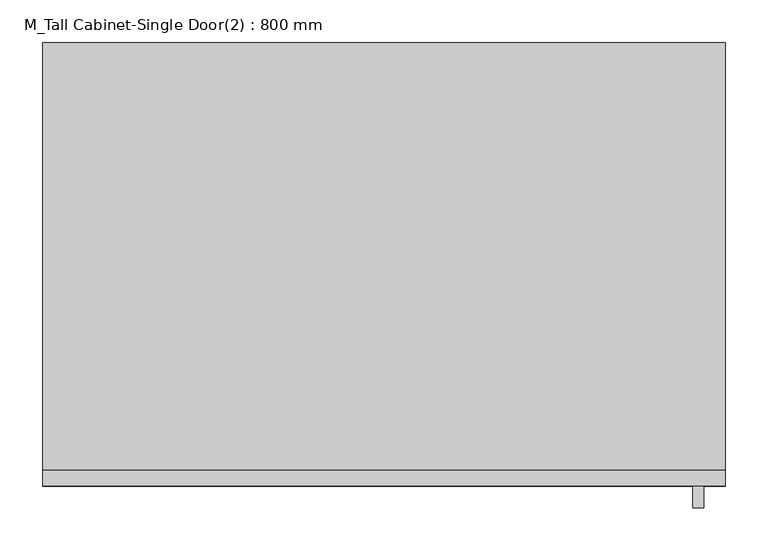
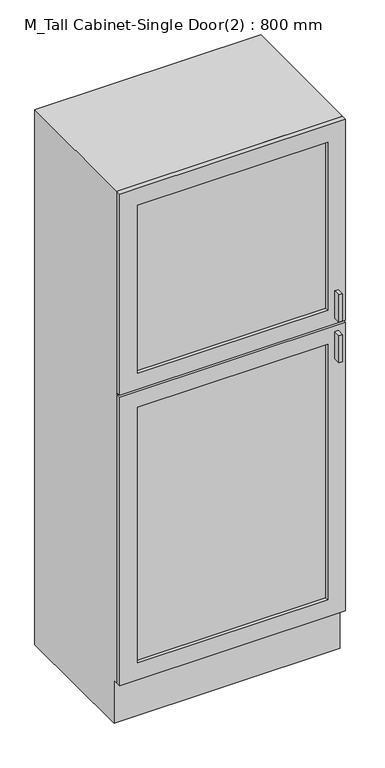
"""IFC4 building model written with IfcOpenShell, lengths in millimetres: furniture geometry, M_Tall Cabinet-Single Door(2) : 800 mm."""

from ifc_helpers import new_model, si_unit, frame, origin, place, context, project, spatial, polyline, outline, extrude, faceted_brep, source, transform, mapped, element, save


def m_tall_cabinet_single_door_2_800_mm_91498984(model_context):
    return source(origin(), model_context, "Body", "SolidModel", [
        faceted_brep([(418.7377049, -500.95, 161.5875), (418.7377049, -500.95, 2000.0), (-381.2622951, -500.95, 2000.0), (-381.2622951, -500.95, 161.5875), (399.6877049, -500.95, 1980.95), (399.6877049, -500.95, 180.6375), (-362.2122951, -500.95, 180.6375), (-362.2122951, -500.95, 1980.95), (-381.2622951, 0.0, 2000.0), (418.7377049, 0.0, 2000.0), (418.7377049, 0.0, 0.0), (-381.2622951, 0.0, 0.0), (399.6877049, 0.0, 1980.95), (-362.2122951, 0.0, 1980.95), (-362.2122951, 0.0, 180.6375), (399.6877049, 0.0, 180.6375), (418.7377049, -485.0, 161.5875), (418.7377049, -485.0, 0.0), (-381.2622951, -485.0, 0.0), (-381.2622951, -485.0, 161.5875)], [[[0, 1, 2, 3], [4, 5, 6, 7]], [[8, 9, 10, 11], [12, 13, 14, 15]], [[1, 0, 16, 17, 10, 9]], [[2, 1, 9, 8]], [[3, 2, 8, 11, 18, 19]], [[0, 3, 19, 16]], [[5, 4, 12, 15]], [[6, 5, 15, 14]], [[7, 6, 14, 13]], [[4, 7, 13, 12]], [[10, 17, 18, 11]], [[18, 17, 16, 19]]]),
        extrude(outline(polyline([(393.3377049, -545.4), (380.8054733, -545.4), (380.8054733, -520.0), (393.3377049, -520.0), (393.3377049, -545.4)])), frame((0.0, 0.0, 1269.9480367), z_axis=(0.0, 0.0, 1.0), x_axis=(1.0, 0.0, 0.0)), (0.0, 0.0, 1.0), 101.6),
        extrude(outline(polyline([(393.3377049, -545.4), (380.8054733, -545.4), (380.8054733, -520.0), (393.3377049, -520.0), (393.3377049, -545.4)])), frame((0.0, 0.0, 1117.5480367), z_axis=(0.0, 0.0, 1.0), x_axis=(1.0, 0.0, 0.0)), (0.0, 0.0, 1.0), 101.6),
        extrude(outline(polyline([(355.2377049, -507.3), (-317.7622951, -507.3), (-317.7622951, -500.95), (355.2377049, -500.95), (355.2377049, -507.3)])), frame((0.0, 0.0, 1308.0480367), z_axis=(0.0, 0.0, 1.0), x_axis=(1.0, 0.0, 0.0)), (0.0, 0.0, 1.0), 628.4519633),
        extrude(outline(polyline([(355.2377049, -507.3), (-317.7622951, -507.3), (-317.7622951, -500.95), (355.2377049, -500.95), (355.2377049, -507.3)])), frame((0.0, 0.0, 225.0875), z_axis=(0.0, 0.0, 1.0), x_axis=(1.0, 0.0, 0.0)), (0.0, 0.0, 1.0), 955.9605367),
        extrude(outline(polyline([(2000.0, 418.7377049), (2000.0, -381.2622951), (1247.7230367, -381.2622951), (1247.7230367, 418.7377049), (2000.0, 418.7377049)]), holes=[polyline([(1936.5, 355.2377049), (1308.0480367, 355.2377049), (1308.0480367, -317.7622951), (1936.5, -317.7622951), (1936.5, 355.2377049)])]), frame((0.0, -520.0, 0.0), z_axis=(0.0, 1.0, 0.0), x_axis=(0.0, 0.0, 1.0)), (0.0, 0.0, 1.0), 19.05),
        extrude(outline(polyline([(161.5875, 418.7377049), (1241.3730367, 418.7377049), (1241.3730367, -381.2622951), (161.5875, -381.2622951), (161.5875, 418.7377049)]), holes=[polyline([(1181.0480367, 355.2377049), (225.0875, 355.2377049), (225.0875, -317.7622951), (1181.0480367, -317.7622951), (1181.0480367, 355.2377049)])]), frame((0.0, -520.0, 0.0), z_axis=(0.0, 1.0, 0.0), x_axis=(0.0, 0.0, 1.0)), (0.0, 0.0, 1.0), 19.05),
        extrude(outline(polyline([(399.6877049, -19.05), (-362.2122951, -19.05), (-362.2122951, 0.0), (399.6877049, 0.0), (399.6877049, -19.05)])), frame((0.0, 0.0, 180.6375), z_axis=(0.0, 0.0, 1.0), x_axis=(1.0, 0.0, 0.0)), (0.0, 0.0, 1.0), 1800.3125),
    ])


if __name__ == "__main__":
    model = new_model("IFC4")
    model_context = context("Model", 3, world=origin())
    ifc_project = project(units=[si_unit("LENGTHUNIT", "METRE", prefix="MILLI")], contexts=[model_context])
    site = spatial("IfcSite", under=ifc_project)
    building = spatial("IfcBuilding", under=site)
    placement = place(None, origin())
    m_tall_cabinet_single_door_2_800_mm_shape = m_tall_cabinet_single_door_2_800_mm_91498984(model_context)
    element("IfcFurniture", 1, ObjectType="M_Tall Cabinet-Single Door(2) : 800 mm", at=placement, inside=building, context=model_context, shape_type="MappedRepresentation", body=[
        mapped(m_tall_cabinet_single_door_2_800_mm_shape, transform((0.0, 0.0, 0.0), x_axis=(1.0, 0.0, 0.0), y_axis=(0.0, 1.0, 0.0), z_axis=(0.0, 0.0, 1.0))),
    ])
    save(model, "model.ifc")

# Revit data of these elements
# Type "M_Tall Cabinet-Single Door(2) : 800 mm"
#   Manufacturer = "Manufacturer"
#   Finish = "Finish"
#   Construction Type = "Construction Type"
#   AccessibilityPerformance = "AccessibilityPerformance"
#   CodePerformance = "CodePerformance"
#   Area = "Area"
#   Color = "Color"
#   Constituents = "Constituents"
#   Features = "Features"
#   Finish = "Finish"
#   Grade = "Grade"
#   Material = "Material"
#   ModelReference = "ModelReference"
#   NominalHeight = "NominalHeight"
#   NominalLength = "NominalLength"
#   NominalWidth = "NominalWidth"
#   ProductionYear = "ProductionYear"
#   Reference = "Reference"
#   Shape = "Shape"
#   Size = "Size"
#   SustainabilityPerformance = "SustainabilityPerformance"
#   WarrantyDescription = "WarrantyDescription"
#   WarrantyDurationLabor = "WarrantyDurationLabor"
#   WarrantyDurationParts = "WarrantyDurationParts"
#   WarrantyGuarantorLabor = "WarrantyGuarantorLabor"
#   WarrantyGuarantorParts = "WarrantyGuarantorParts"
#   ExpectedLife = "ExpectedLife"
#   ReplacementCost = "ReplacementCost"
#   AssetAccountingType = "FIXED"
#   ModelLabel = "ModelLabel"
#   Depth = 0.520 m
#   Height = 2.000 m
#   Plinth Depth = 0.035 m
#   Plinth Height = 0.160 m
#   Width = 0.800 m
#   Cabinet Material = none
#   Door/Drawer Material = none
#   Handle Material = Cabinets - Handles
#   Panel Material = Cabinets - Panel
# Element 1 (IfcFurniture, "M_Tall Cabinet-Single Door(2) : 800 mm")
#   Materials on its faces: "Cabinets", "Cabinets - Handles", "Cabinets - Panel"
# Materials
#   "Cabinets - Handles": class "Metal", colour RGB 57 57 57, transparency 0
#   "Cabinets - Panel": class "Miscellaneous", colour RGB 249 249 249, transparency 0
#   "Cabinets": class "Miscellaneous", colour RGB 249 249 249, transparency 0
